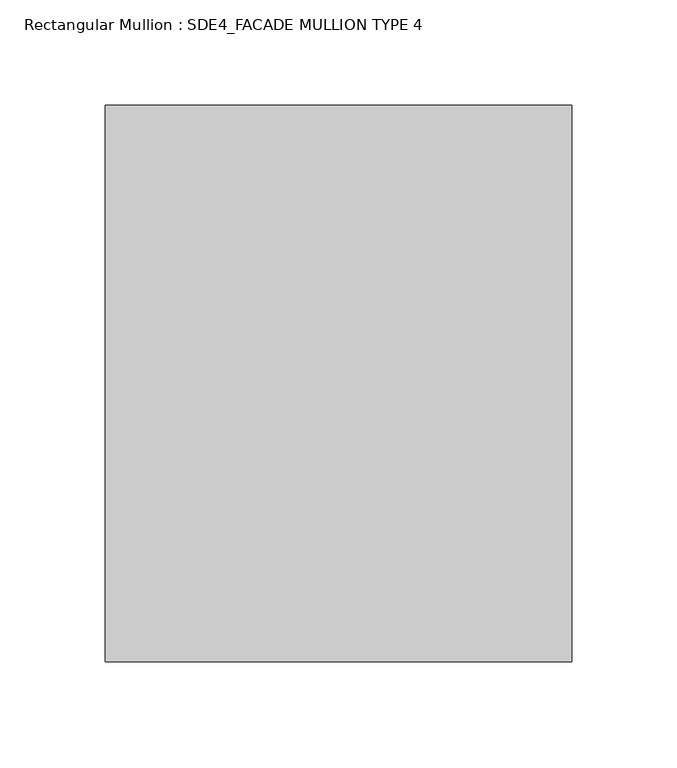
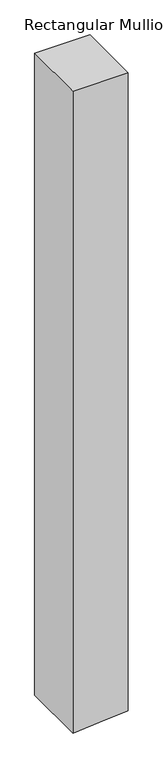
"""IFC4 building model written with IfcOpenShell, lengths in millimetres: member geometry, Rectangular Mullion : SDE4_FACADE MULLION TYPE 4."""

import ifcopenshell
import ifcopenshell.guid

model = None  # the IFC model being written
_history = None  # IfcOwnerHistory: only IFC2X3 demands one
_inside = {}  # id of a spatial element -> (the spatial element, [elements in it])
_under = {}  # id of a project, library or spatial element -> (it, [spatial elements below it])
_declared = {}  # id of a project -> (the project, [libraries it declares])
_typed = {}  # id of a type object -> (the type object, [elements of that type])
_made_of = {}  # id of a material, layer set ... -> (it, [elements and type objects made of it])


def new_model(schema):
    """Start an empty IFC model of exactly this schema.

    Asked for "IFC4X3", IfcOpenShell would pick the latest addendum, in which some entities
    have other attributes; the version numbers below select the first issue.
    IFC2X3 requires an IfcOwnerHistory on every rooted entity: one is made here for all.
    """
    global model, _history
    if schema == "IFC4X3":
        model = ifcopenshell.file(schema_version=(4, 3, 0, 0))
    else:
        model = ifcopenshell.file(schema=schema)
    _inside.clear()
    _under.clear()
    _declared.clear()
    _typed.clear()
    _made_of.clear()
    _history = None
    if model.schema == "IFC2X3":
        org = make("IfcOrganization", Name="unknown")
        user = make(
            "IfcPersonAndOrganization",
            ThePerson=make("IfcPerson", FamilyName="unknown"),
            TheOrganization=org,
        )
        app = make(
            "IfcApplication",
            ApplicationDeveloper=org,
            Version="unknown",
            ApplicationFullName="unknown",
            ApplicationIdentifier="unknown",
        )
        _history = make(
            "IfcOwnerHistory",
            OwningUser=user,
            OwningApplication=app,
            ChangeAction="ADDED",
            CreationDate=0,
        )
    return model


def make(cls, **values):
    """One entity of the class cls with the attributes given. An attribute that is None is left unset."""
    return model.create_entity(
        cls, **{name: value for name, value in values.items() if value is not None}
    )


def rooted(cls, **values):
    """An entity with a GlobalId (a new one), such as an element, a storey or a relation."""
    return make(cls, GlobalId=ifcopenshell.guid.new(), OwnerHistory=_history, **values)


def si_unit(unit_type, name, prefix=None):
    """IfcSIUnit, for example si_unit("LENGTHUNIT", "METRE", prefix="MILLI")."""
    return make("IfcSIUnit", UnitType=unit_type, Prefix=prefix, Name=name)


def assignment(units):
    """IfcUnitAssignment: the units of a project."""
    return None if units is None else make("IfcUnitAssignment", Units=units)


def point(xyz):
    """IfcCartesianPoint."""
    return None if xyz is None else make("IfcCartesianPoint", Coordinates=xyz)


def direction(xyz):
    """IfcDirection."""
    return None if xyz is None else make("IfcDirection", DirectionRatios=xyz)


def frame(location, z_axis=None, x_axis=None):
    """IfcAxis2Placement3D, a coordinate frame: its origin and axes. An axis left out is left unset."""
    return make(
        "IfcAxis2Placement3D",
        Location=point(location),
        Axis=direction(z_axis),
        RefDirection=direction(x_axis),
    )


def origin():
    """The frame at (0, 0, 0) with its axes left unset."""
    return frame((0.0, 0.0, 0.0))


def place(relative_to, where):
    """IfcLocalPlacement: puts the frame where relative to a parent placement (None: the world)."""
    return make(
        "IfcLocalPlacement", PlacementRelTo=relative_to, RelativePlacement=where
    )


def context(
    kind, dimensions, precision=None, world=None, true_north=None, identifier=None
):
    """IfcGeometricRepresentationContext, for example the 3D "Model" context."""
    return make(
        "IfcGeometricRepresentationContext",
        ContextIdentifier=identifier,
        ContextType=kind,
        CoordinateSpaceDimension=dimensions,
        Precision=precision,
        WorldCoordinateSystem=world,
        TrueNorth=true_north,
    )


def project(units=None, contexts=None):
    """IfcProject with its units and contexts."""
    return rooted(
        "IfcProject",
        Name="project",
        RepresentationContexts=contexts,
        UnitsInContext=assignment(units),
    )


def spatial(cls, under=None, at=None, **own):
    """A site, building, storey or space (cls), placed at a placement, below another one or the project."""
    s = rooted(cls, ObjectPlacement=at, **own)
    if under is not None:
        _under.setdefault(under.id(), (under, []))[1].append(s)
    return s


def polyline(points):
    """IfcPolyline through the points."""
    return make("IfcPolyline", Points=[point(p) for p in points])


def outline(outer, holes=None, kind="AREA"):
    """IfcArbitraryClosedProfileDef: a profile drawn as a closed curve; with holes, ...WithVoids."""
    if holes is None:
        return make("IfcArbitraryClosedProfileDef", ProfileType=kind, OuterCurve=outer)
    return make(
        "IfcArbitraryProfileDefWithVoids",
        ProfileType=kind,
        OuterCurve=outer,
        InnerCurves=holes,
    )


def extrude(swept, where, along, depth):
    """IfcExtrudedAreaSolid: the profile swept, set in the frame where, extruded along a direction by depth."""
    return make(
        "IfcExtrudedAreaSolid",
        SweptArea=swept,
        Position=where,
        ExtrudedDirection=direction(along),
        Depth=depth,
    )


def shape(context_of_items, identifier, shape_type, items):
    """IfcShapeRepresentation: the items that make up one representation, for example the "Body"."""
    return make(
        "IfcShapeRepresentation",
        ContextOfItems=context_of_items,
        RepresentationIdentifier=identifier,
        RepresentationType=shape_type,
        Items=items,
    )


def source(mapping_origin, context_of_items, identifier, shape_type, items):
    """IfcRepresentationMap: a shape defined once, which mapped items show again and again."""
    return make(
        "IfcRepresentationMap",
        MappingOrigin=mapping_origin,
        MappedRepresentation=shape(context_of_items, identifier, shape_type, items),
    )


def transform(
    local_origin,
    x_axis=None,
    y_axis=None,
    z_axis=None,
    scale=None,
    scale2=None,
    scale3=None,
    uniform=True,
):
    """IfcCartesianTransformationOperator3D, or its non-uniform kind. x_axis, y_axis, z_axis: its Axis1, 2, 3."""
    if uniform:
        return make(
            "IfcCartesianTransformationOperator3D",
            Axis1=direction(x_axis),
            Axis2=direction(y_axis),
            LocalOrigin=point(local_origin),
            Scale=scale,
            Axis3=direction(z_axis),
        )
    return make(
        "IfcCartesianTransformationOperator3DnonUniform",
        Axis1=direction(x_axis),
        Axis2=direction(y_axis),
        LocalOrigin=point(local_origin),
        Scale=scale,
        Axis3=direction(z_axis),
        Scale2=scale2,
        Scale3=scale3,
    )


def mapped(mapping_source, mapping_target):
    """IfcMappedItem: shows the shape of a source again, moved by a transform."""
    return make(
        "IfcMappedItem", MappingSource=mapping_source, MappingTarget=mapping_target
    )


def made_of(thing, what):
    """Note that an element or type object is made of a material, layer set ...; save() writes the relation."""
    if what is not None:
        _made_of.setdefault(what.id(), (what, []))[1].append(thing)
    return thing


def element(
    cls,
    number,
    at=None,
    inside=None,
    cuts=None,
    type_object=None,
    material=None,
    context=None,
    identifier="Body",
    shape_type=None,
    held_by="IfcProductDefinitionShape",
    body=None,
    shapes=None,
    **own,
):
    """One element of the class cls, such as IfcWall. Its Tag is "e" and its number.

    at: its placement. inside: the storey or other place that contains it. cuts: it is an
    opening in that element (IfcRelVoidsElement). A single representation is given by context,
    identifier, shape_type and body (its items); several are given by shapes. held_by: the class
    of the entity that holds the representations. save() writes the other relations.
    """
    e = rooted(cls, Tag="e%d" % number, ObjectPlacement=at, **own)
    if body is not None:
        shapes = [shape(context, identifier, shape_type, body)]
    if shapes is not None:
        e.Representation = make(held_by, Representations=shapes)
    if inside is not None:
        _inside.setdefault(inside.id(), (inside, []))[1].append(e)
    if cuts is not None:
        rooted(
            "IfcRelVoidsElement", RelatingBuildingElement=cuts, RelatedOpeningElement=e
        )
    if type_object is not None:
        _typed.setdefault(type_object.id(), (type_object, []))[1].append(e)
    return made_of(e, material)


def aggregate(whole, parts):
    """IfcRelAggregates: a whole, such as a stair, and the parts it consists of."""
    return rooted("IfcRelAggregates", RelatingObject=whole, RelatedObjects=parts)


def save(model, path):
    """Write the relations noted so far, then the file.

    IfcRelAggregates (storeys below a building ...), IfcRelContainedInSpatialStructure (elements
    in a storey), IfcRelDefinesByType, IfcRelAssociatesMaterial and IfcRelDeclares: one each for
    every whole, place, type object, material and project.
    """
    for whole, parts in _under.values():
        aggregate(whole, parts)
    for where, things in _inside.values():
        rooted(
            "IfcRelContainedInSpatialStructure",
            RelatedElements=things,
            RelatingStructure=where,
        )
    for kind, things in _typed.values():
        rooted("IfcRelDefinesByType", RelatedObjects=things, RelatingType=kind)
    for what, things in _made_of.values():
        rooted("IfcRelAssociatesMaterial", RelatedObjects=things, RelatingMaterial=what)
    for by, libraries in _declared.values():
        rooted("IfcRelDeclares", RelatingContext=by, RelatedDefinitions=libraries)
    model.write(path)


def rectangular_mullion_sde4_facade_mullion_type_4_53a8cb0c(model_context):
    return source(origin(), model_context, "Body", "SweptSolid", [
        extrude(outline(polyline([(0.0, 111.0), (0.0, -111.0), (-2725.9162826, -111.0), (-2717.6438427, -3.056508), (-2708.9029211, 111.0), (0.0, 111.0)])), frame((0.0, -132.5, 0.0), z_axis=(0.0, 1.0, 0.0), x_axis=(0.0, 0.0, 1.0)), (0.0, 0.0, 1.0), 265.0),
    ])


if __name__ == "__main__":
    model = new_model("IFC4")
    model_context = context("Model", 3, world=origin())
    ifc_project = project(units=[si_unit("LENGTHUNIT", "METRE", prefix="MILLI")], contexts=[model_context])
    site = spatial("IfcSite", under=ifc_project)
    building = spatial("IfcBuilding", under=site)
    placement = place(None, origin())
    rectangular_mullion_sde4_facade_mullion_type_4_shape = rectangular_mullion_sde4_facade_mullion_type_4_53a8cb0c(model_context)
    element("IfcMember", 1, ObjectType="Rectangular Mullion : SDE4_FACADE MULLION TYPE 4", at=placement, inside=building, context=model_context, shape_type="MappedRepresentation", body=[
        mapped(rectangular_mullion_sde4_facade_mullion_type_4_shape, transform((0.0, 0.0, 0.0), x_axis=(1.0, 0.0, 0.0), y_axis=(0.0, 1.0, 0.0), z_axis=(0.0, 0.0, 1.0))),
    ])
    save(model, "model.ifc")

# Revit data of these elements
# Type "Rectangular Mullion : SDE4_FACADE MULLION TYPE 4"
#   built-in parameter 1007322 = 0.869423 (stored number, unit not read)
#   built-in parameter 1007321 = 0.364173 (stored number, unit not read)
#   built-in parameter 1007320 = 0.364173 (stored number, unit not read)
